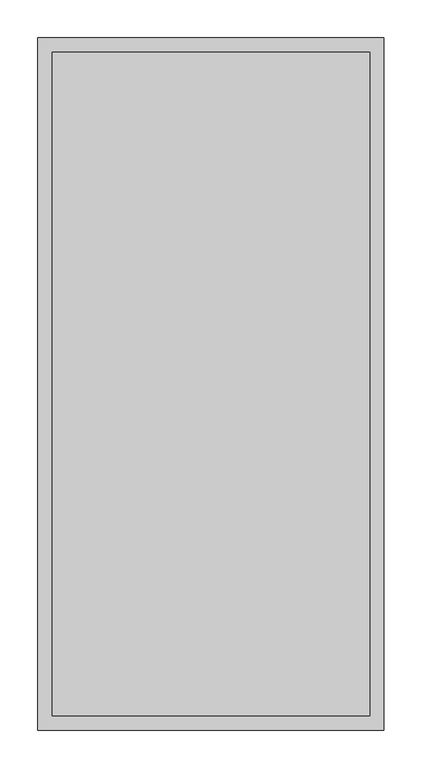
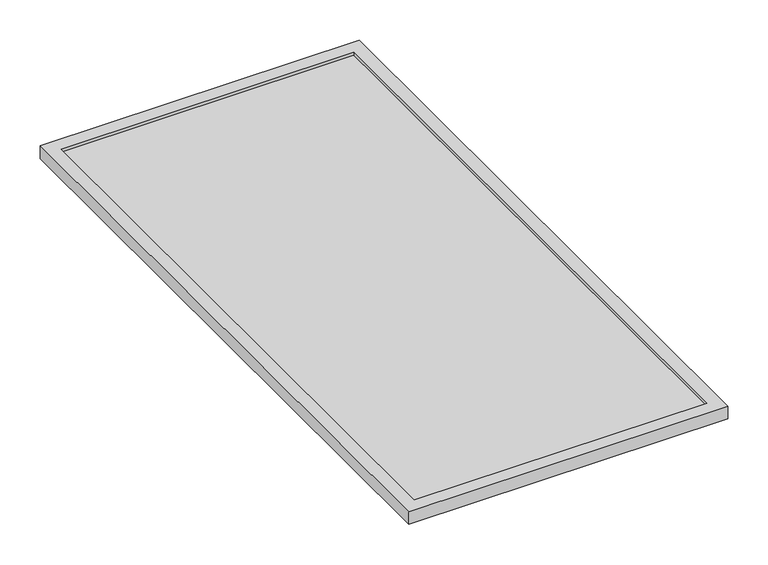
"""IFC4 building model written with IfcOpenShell, lengths in millimetres: proxy geometry, Bradley-Washroom_Accessories-Mirrors-780_Custom : Bradley-Washroom_Accessories-Mirrors-780_Custom."""

from ifc_helpers import new_model, si_unit, frame, origin, place, context, project, spatial, polyline, outline, extrude, faceted_brep, source, transform, mapped, element, save


def specialty_equipment_075658ae(model_context):
    return source(origin(), model_context, "Body", "SolidModel", [
        extrude(outline(polyline([(209.55, -438.15), (-209.55, -438.15), (-209.55, 438.15), (209.55, 438.15), (209.55, -438.15)])), frame((0.0, 0.0, 9.525), z_axis=(0.0, 0.0, 1.0), x_axis=(1.0, 0.0, 0.0)), (0.0, 0.0, 1.0), 4.7625),
        faceted_brep([(228.6, -457.2, 19.05), (228.6, 457.2, 19.05), (-228.6, 457.2, 19.05), (-228.6, -457.2, 19.05), (-209.55, -438.15, 19.05), (-209.55, 438.15, 19.05), (209.55, 438.15, 19.05), (209.55, -438.15, 19.05), (228.6, -457.2, 0.0), (-228.6, -457.2, 0.0), (-228.6, 457.2, 0.0), (228.6, 457.2, 0.0), (209.55, -438.15, 9.525), (209.55, 438.15, 9.525), (-209.55, 438.15, 9.525), (-209.55, -438.15, 9.525)], [[[0, 1, 2, 3], [4, 5, 6, 7]], [[8, 9, 10, 11]], [[3, 9, 8, 0]], [[2, 10, 9, 3]], [[1, 11, 10, 2]], [[0, 8, 11, 1]], [[12, 13, 14, 15]], [[15, 4, 7, 12]], [[14, 5, 4, 15]], [[13, 6, 5, 14]], [[12, 7, 6, 13]]]),
    ])


if __name__ == "__main__":
    model = new_model("IFC4")
    model_context = context("Model", 3, world=origin())
    ifc_project = project(units=[si_unit("LENGTHUNIT", "METRE", prefix="MILLI")], contexts=[model_context])
    site = spatial("IfcSite", under=ifc_project)
    building = spatial("IfcBuilding", under=site)
    placement = place(None, origin())
    specialty_equipment_shape = specialty_equipment_075658ae(model_context)
    element("IfcBuildingElementProxy", 1, Name="Bradley-Washroom_Accessories-Mirrors-780_Custom : Bradley-Washroom_Accessories-Mirrors-780_Custom", ObjectType="Bradley-Washroom_Accessories-Mirrors-780_Custom : Bradley-Washroom_Accessories-Mirrors-780_Custom", at=placement, inside=building, context=model_context, shape_type="MappedRepresentation", body=[
        mapped(specialty_equipment_shape, transform((0.0, 0.0, 0.0), x_axis=(1.0, 0.0, 0.0), y_axis=(0.0, 1.0, 0.0), z_axis=(0.0, 0.0, 1.0))),
    ])
    save(model, "model.ifc")

# Revit data of these elements
# Project information
#   Project Issue Date = "07/20/2015"
#   Project Status = "Project Status"
#   Client Name = "Xcel"
#   Project Address = "Enter address here"
#   Project Name = "Xcel Sports Complex - Jefferson, WI"
#   Project Number = "Project Number"
# Type "Bradley-Washroom_Accessories-Mirrors-780_Custom : Bradley-Washroom_Accessories-Mirrors-780_Custom"
#   Warranty Information = "Complete unit, excepting mirrors warranted for one year.\r\n Stainless steel mirror frames for fifteen years.\r\n Plate glass mirrors for fifteen years.\r\n This warranty does not cover installation or any other labor charges and does not apply to any units,\r\n which have been damaged by accident, abuse, improper installation, improper maintenance, or altered in any way."
#   Version = "1.0"
#   URL = "http://www.bradleycorp.com/"
#   Type Comments = "ERROR - If you are able to see this message you haven't loaded this  family correctly."
#   OmniClass Title = "Mirrors"
#   OmniClass Code = "23.40.95.17.17"
#   Modeling Code = ""
#   Model = "ERROR - If you are able to see this message you haven't loaded this  family correctly."
#   MasterFormat Title = "Commercial Toilet Accessories"
#   MasterFormat Number = "10 28 13. 13"
#   Manufacturer = "Bradley Corporation"
#   Keynote = "M08831300.01"
#   Industry Standards = "ASTM C 1036"
#   Fire Rating = "n/a"
#   Dimensional Limits [instance default] = "Either Width or Hight must be over 25\""
#   Description = "ERROR - If you are able to see this message you haven't loaded this  family correctly."
#   Copyright = "This Model Data is Property of Bradley Corporation"
#   Buy American Act = "Yes"
#   Assembly Code = "C1030900"
#   ADA Compliant = "Yes"
#   Width [instance default] = 1' - 6"
#   Total Width [instance default] = 1' - 6"
#   Total Height [instance default] = 3' - 0"
#   Height [instance default] = 3' - 0"
#   Depth [instance default] = 0' - 0 3/4"
#   Default Elevation = 3' - 4"
#   Reflective Material = Glass - Bradley Corp - BradEX - Polished Float Mirror
#   Frame Material = Bradley Corp Stainless Steel - Satin
# Element 1 (IfcBuildingElementProxy, "Bradley-Washroom_Accessories-Mirrors-780_Custom : Bradley-Washroom_Accessories-Mirrors-780_Custom")
#   Materials on its faces: "Bradley Corp Stainless Steel - Satin", "Glass - Bradley Corp - BradEX - Polished Float Mirror"
# Materials
#   "Glass - Bradley Corp - BradEX - Polished Float Mirror": class "Glass", colour RGB 221 230 232, transparency 0, Manufacturer = "Bradley Corporation", URL = "www.bradleycorp.com", Description = "Stainless Steel - Satin Finish", Cost = 0
#   "Bradley Corp Stainless Steel - Satin": class "Metal", colour RGB 189 187 185, transparency 0, Manufacturer = "Bradley Corporation", URL = "www.bradleycorp.com", Description = "Stainless Steel - Satin Finish", Cost = 0
